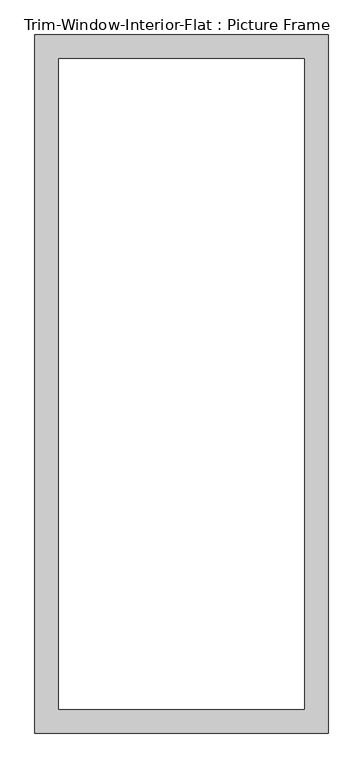
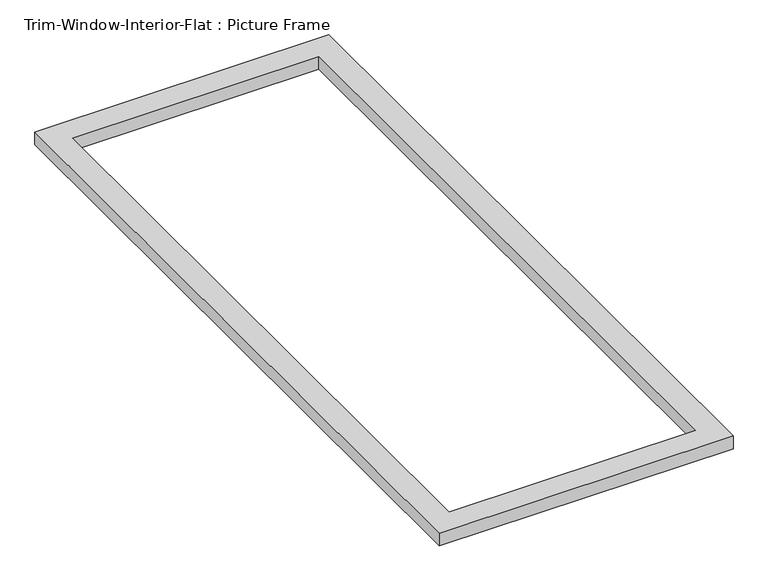
"""IFC4 building model written with IfcOpenShell, lengths in millimetres: proxy geometry, Trim-Window-Interior-Flat : Picture Frame."""

import ifcopenshell
import ifcopenshell.guid

model = None  # the IFC model being written
_history = None  # IfcOwnerHistory: only IFC2X3 demands one
_inside = {}  # id of a spatial element -> (the spatial element, [elements in it])
_under = {}  # id of a project, library or spatial element -> (it, [spatial elements below it])
_declared = {}  # id of a project -> (the project, [libraries it declares])
_typed = {}  # id of a type object -> (the type object, [elements of that type])
_made_of = {}  # id of a material, layer set ... -> (it, [elements and type objects made of it])


def new_model(schema):
    """Start an empty IFC model of exactly this schema.

    Asked for "IFC4X3", IfcOpenShell would pick the latest addendum, in which some entities
    have other attributes; the version numbers below select the first issue.
    IFC2X3 requires an IfcOwnerHistory on every rooted entity: one is made here for all.
    """
    global model, _history
    if schema == "IFC4X3":
        model = ifcopenshell.file(schema_version=(4, 3, 0, 0))
    else:
        model = ifcopenshell.file(schema=schema)
    _inside.clear()
    _under.clear()
    _declared.clear()
    _typed.clear()
    _made_of.clear()
    _history = None
    if model.schema == "IFC2X3":
        org = make("IfcOrganization", Name="unknown")
        user = make(
            "IfcPersonAndOrganization",
            ThePerson=make("IfcPerson", FamilyName="unknown"),
            TheOrganization=org,
        )
        app = make(
            "IfcApplication",
            ApplicationDeveloper=org,
            Version="unknown",
            ApplicationFullName="unknown",
            ApplicationIdentifier="unknown",
        )
        _history = make(
            "IfcOwnerHistory",
            OwningUser=user,
            OwningApplication=app,
            ChangeAction="ADDED",
            CreationDate=0,
        )
    return model


def make(cls, **values):
    """One entity of the class cls with the attributes given. An attribute that is None is left unset."""
    return model.create_entity(
        cls, **{name: value for name, value in values.items() if value is not None}
    )


def rooted(cls, **values):
    """An entity with a GlobalId (a new one), such as an element, a storey or a relation."""
    return make(cls, GlobalId=ifcopenshell.guid.new(), OwnerHistory=_history, **values)


def si_unit(unit_type, name, prefix=None):
    """IfcSIUnit, for example si_unit("LENGTHUNIT", "METRE", prefix="MILLI")."""
    return make("IfcSIUnit", UnitType=unit_type, Prefix=prefix, Name=name)


def assignment(units):
    """IfcUnitAssignment: the units of a project."""
    return None if units is None else make("IfcUnitAssignment", Units=units)


def point(xyz):
    """IfcCartesianPoint."""
    return None if xyz is None else make("IfcCartesianPoint", Coordinates=xyz)


def direction(xyz):
    """IfcDirection."""
    return None if xyz is None else make("IfcDirection", DirectionRatios=xyz)


def frame(location, z_axis=None, x_axis=None):
    """IfcAxis2Placement3D, a coordinate frame: its origin and axes. An axis left out is left unset."""
    return make(
        "IfcAxis2Placement3D",
        Location=point(location),
        Axis=direction(z_axis),
        RefDirection=direction(x_axis),
    )


def origin():
    """The frame at (0, 0, 0) with its axes left unset."""
    return frame((0.0, 0.0, 0.0))


def origin_with_axes():
    """The frame at (0, 0, 0) with the z axis (0, 0, 1) and the x axis (1, 0, 0) written out."""
    return frame((0.0, 0.0, 0.0), z_axis=(0.0, 0.0, 1.0), x_axis=(1.0, 0.0, 0.0))


def place(relative_to, where):
    """IfcLocalPlacement: puts the frame where relative to a parent placement (None: the world)."""
    return make(
        "IfcLocalPlacement", PlacementRelTo=relative_to, RelativePlacement=where
    )


def context(
    kind, dimensions, precision=None, world=None, true_north=None, identifier=None
):
    """IfcGeometricRepresentationContext, for example the 3D "Model" context."""
    return make(
        "IfcGeometricRepresentationContext",
        ContextIdentifier=identifier,
        ContextType=kind,
        CoordinateSpaceDimension=dimensions,
        Precision=precision,
        WorldCoordinateSystem=world,
        TrueNorth=true_north,
    )


def project(units=None, contexts=None):
    """IfcProject with its units and contexts."""
    return rooted(
        "IfcProject",
        Name="project",
        RepresentationContexts=contexts,
        UnitsInContext=assignment(units),
    )


def spatial(cls, under=None, at=None, **own):
    """A site, building, storey or space (cls), placed at a placement, below another one or the project."""
    s = rooted(cls, ObjectPlacement=at, **own)
    if under is not None:
        _under.setdefault(under.id(), (under, []))[1].append(s)
    return s


def polyline(points):
    """IfcPolyline through the points."""
    return make("IfcPolyline", Points=[point(p) for p in points])


def outline(outer, holes=None, kind="AREA"):
    """IfcArbitraryClosedProfileDef: a profile drawn as a closed curve; with holes, ...WithVoids."""
    if holes is None:
        return make("IfcArbitraryClosedProfileDef", ProfileType=kind, OuterCurve=outer)
    return make(
        "IfcArbitraryProfileDefWithVoids",
        ProfileType=kind,
        OuterCurve=outer,
        InnerCurves=holes,
    )


def extrude(swept, where, along, depth):
    """IfcExtrudedAreaSolid: the profile swept, set in the frame where, extruded along a direction by depth."""
    return make(
        "IfcExtrudedAreaSolid",
        SweptArea=swept,
        Position=where,
        ExtrudedDirection=direction(along),
        Depth=depth,
    )


def shape(context_of_items, identifier, shape_type, items):
    """IfcShapeRepresentation: the items that make up one representation, for example the "Body"."""
    return make(
        "IfcShapeRepresentation",
        ContextOfItems=context_of_items,
        RepresentationIdentifier=identifier,
        RepresentationType=shape_type,
        Items=items,
    )


def source(mapping_origin, context_of_items, identifier, shape_type, items):
    """IfcRepresentationMap: a shape defined once, which mapped items show again and again."""
    return make(
        "IfcRepresentationMap",
        MappingOrigin=mapping_origin,
        MappedRepresentation=shape(context_of_items, identifier, shape_type, items),
    )


def transform(
    local_origin,
    x_axis=None,
    y_axis=None,
    z_axis=None,
    scale=None,
    scale2=None,
    scale3=None,
    uniform=True,
):
    """IfcCartesianTransformationOperator3D, or its non-uniform kind. x_axis, y_axis, z_axis: its Axis1, 2, 3."""
    if uniform:
        return make(
            "IfcCartesianTransformationOperator3D",
            Axis1=direction(x_axis),
            Axis2=direction(y_axis),
            LocalOrigin=point(local_origin),
            Scale=scale,
            Axis3=direction(z_axis),
        )
    return make(
        "IfcCartesianTransformationOperator3DnonUniform",
        Axis1=direction(x_axis),
        Axis2=direction(y_axis),
        LocalOrigin=point(local_origin),
        Scale=scale,
        Axis3=direction(z_axis),
        Scale2=scale2,
        Scale3=scale3,
    )


def mapped(mapping_source, mapping_target):
    """IfcMappedItem: shows the shape of a source again, moved by a transform."""
    return make(
        "IfcMappedItem", MappingSource=mapping_source, MappingTarget=mapping_target
    )


def made_of(thing, what):
    """Note that an element or type object is made of a material, layer set ...; save() writes the relation."""
    if what is not None:
        _made_of.setdefault(what.id(), (what, []))[1].append(thing)
    return thing


def element(
    cls,
    number,
    at=None,
    inside=None,
    cuts=None,
    type_object=None,
    material=None,
    context=None,
    identifier="Body",
    shape_type=None,
    held_by="IfcProductDefinitionShape",
    body=None,
    shapes=None,
    **own,
):
    """One element of the class cls, such as IfcWall. Its Tag is "e" and its number.

    at: its placement. inside: the storey or other place that contains it. cuts: it is an
    opening in that element (IfcRelVoidsElement). A single representation is given by context,
    identifier, shape_type and body (its items); several are given by shapes. held_by: the class
    of the entity that holds the representations. save() writes the other relations.
    """
    e = rooted(cls, Tag="e%d" % number, ObjectPlacement=at, **own)
    if body is not None:
        shapes = [shape(context, identifier, shape_type, body)]
    if shapes is not None:
        e.Representation = make(held_by, Representations=shapes)
    if inside is not None:
        _inside.setdefault(inside.id(), (inside, []))[1].append(e)
    if cuts is not None:
        rooted(
            "IfcRelVoidsElement", RelatingBuildingElement=cuts, RelatedOpeningElement=e
        )
    if type_object is not None:
        _typed.setdefault(type_object.id(), (type_object, []))[1].append(e)
    return made_of(e, material)


def aggregate(whole, parts):
    """IfcRelAggregates: a whole, such as a stair, and the parts it consists of."""
    return rooted("IfcRelAggregates", RelatingObject=whole, RelatedObjects=parts)


def save(model, path):
    """Write the relations noted so far, then the file.

    IfcRelAggregates (storeys below a building ...), IfcRelContainedInSpatialStructure (elements
    in a storey), IfcRelDefinesByType, IfcRelAssociatesMaterial and IfcRelDeclares: one each for
    every whole, place, type object, material and project.
    """
    for whole, parts in _under.values():
        aggregate(whole, parts)
    for where, things in _inside.values():
        rooted(
            "IfcRelContainedInSpatialStructure",
            RelatedElements=things,
            RelatingStructure=where,
        )
    for kind, things in _typed.values():
        rooted("IfcRelDefinesByType", RelatedObjects=things, RelatingType=kind)
    for what, things in _made_of.values():
        rooted("IfcRelAssociatesMaterial", RelatedObjects=things, RelatingMaterial=what)
    for by, libraries in _declared.values():
        rooted("IfcRelDeclares", RelatingContext=by, RelatedDefinitions=libraries)
    model.write(path)


def trim_window_interior_flat_picture_frame_35192fdd(model_context):
    return source(origin(), model_context, "Body", "SweptSolid", [
        extrude(outline(polyline([(349.25, 44.45), (349.25, -1619.25), (-349.25, -1619.25), (-349.25, 44.45), (349.25, 44.45)]), holes=[polyline([(292.1, -12.7), (-292.1, -12.7), (-292.1, -1562.1), (292.1, -1562.1), (292.1, -12.7)])]), origin_with_axes(), (0.0, 0.0, 1.0), 31.75),
    ])


if __name__ == "__main__":
    model = new_model("IFC4")
    model_context = context("Model", 3, world=origin())
    ifc_project = project(units=[si_unit("LENGTHUNIT", "METRE", prefix="MILLI")], contexts=[model_context])
    site = spatial("IfcSite", under=ifc_project)
    building = spatial("IfcBuilding", under=site)
    placement = place(None, origin())
    trim_window_interior_flat_picture_frame_shape = trim_window_interior_flat_picture_frame_35192fdd(model_context)
    element("IfcBuildingElementProxy", 1, Name="Trim-Window-Interior-Flat : Picture Frame", ObjectType="Trim-Window-Interior-Flat : Picture Frame", at=placement, inside=building, context=model_context, shape_type="MappedRepresentation", body=[
        mapped(trim_window_interior_flat_picture_frame_shape, transform((0.0, 0.0, 0.0), x_axis=(1.0, 0.0, 0.0), y_axis=(0.0, 1.0, 0.0), z_axis=(0.0, 0.0, 1.0))),
    ])
    save(model, "model.ifc")

# Revit data of these elements
# Type "Trim-Window-Interior-Flat : Picture Frame"
#   Trim Thickness_Picture Frame = 0' - 1 1/4"
#   Trim Width = 0' - 2 1/4"
#   Trim Thickness_with Sill = 0' - 0 3/4"
#   Sill Thickness = 0' - 1 1/4"
#   Opening Width [instance default] = 2' - 0"
#   Opening Height [instance default] = 3' - 0"
#   Default Elevation = 4' - 0"
#   Sill = no
#   Picture Frame = yes
#   Trim Material [instance default] = none
# Element 1 (IfcBuildingElementProxy, "Trim-Window-Interior-Flat : Picture Frame")
#   Opening Height = 5' - 2"
#   Trim Material = Wood - Stained
#   Materials on its faces: "Wood - Stained"
# Materials
#   "Wood - Stained": class "Wood", colour RGB 224 178 126, transparency 0, Cost = 0
